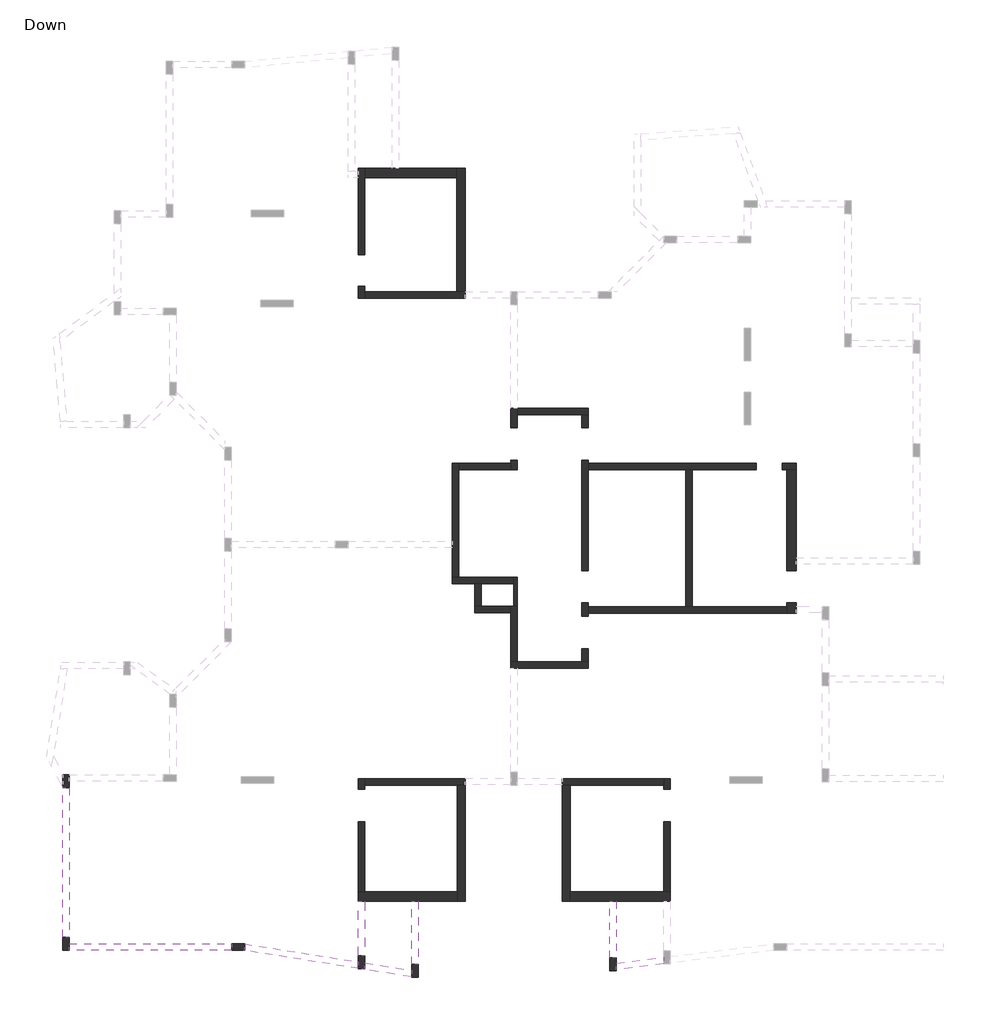
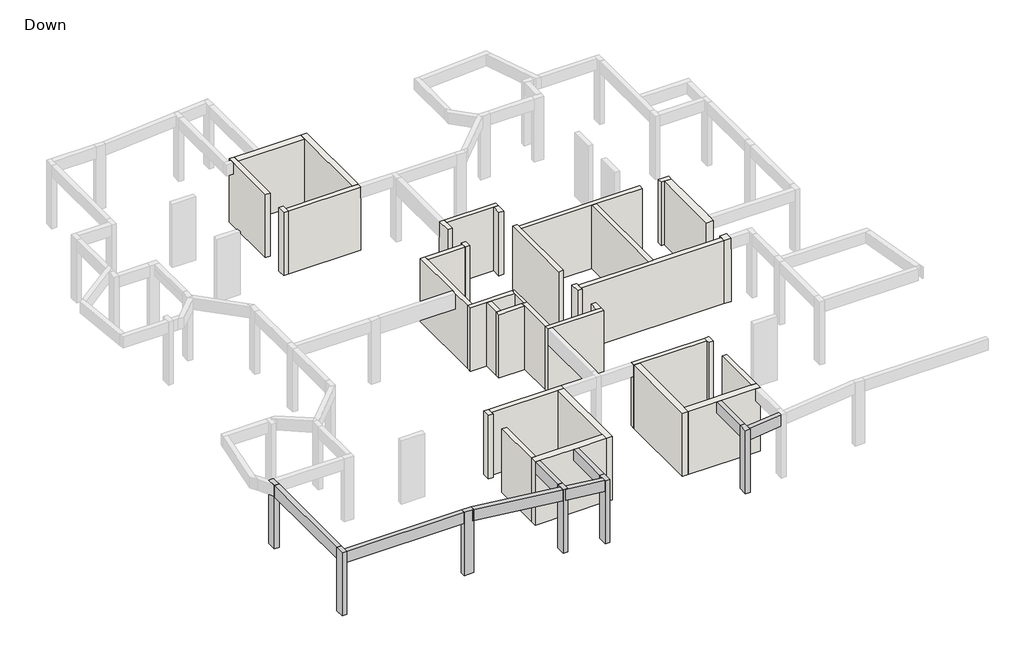
# One storey, part 1 of 3: 36 walls, 8 beams, 6 columns.
# Revit data of these elements (continued)
# Element 33 (IfcWall, "20") (continued)
#   Materials on its faces: "Concrete"
# Element 34 (IfcWall, "20")
#   Comments = ""
#   Mark = "W19"
#   SOFiSTiK_EdgeZones = "W20"
#   SOFiSTiK_AMG_Comments = ""
#   Top Offset = 0 cm
#   Base Offset = 0 cm
#   wall height = 285 cm
#   SOFiSTiK_AMG_Scheduled = yes
#   SOFiSTiK_AMG_Adjusted = yes
#   Phase Created = New Construction
#   Base Constraint = Down
#   Top Constraint = Typical Floor
#   Materials on its faces: "Concrete"
# Element 35 (IfcWall, "20")
#   Comments = ""
#   Mark = "W20"
#   SOFiSTiK_EdgeZones = "W21"
#   SOFiSTiK_AMG_Comments = ""
#   Top Offset = 0 cm
#   Base Offset = 0 cm
#   wall height = 285 cm
#   SOFiSTiK_AMG_Scheduled = yes
#   SOFiSTiK_AMG_Adjusted = yes
#   Phase Created = New Construction
#   Base Constraint = Down
#   Top Constraint = Typical Floor
#   Materials on its faces: "Concrete"
# Element 36 (IfcWall, "20")
#   Comments = ""
#   Mark = "W21"
#   SOFiSTiK_EdgeZones = "W22"
#   SOFiSTiK_AMG_Comments = ""
#   Top Offset = 0 cm
#   Base Offset = 0 cm
#   wall height = 285 cm
#   SOFiSTiK_AMG_Scheduled = yes
#   SOFiSTiK_AMG_Adjusted = yes
#   Phase Created = New Construction
#   Base Constraint = Down
#   Top Constraint = Typical Floor
#   Materials on its faces: "Concrete"
# Element 37 (IfcWall, "20")
#   Comments = ""
#   Mark = "W22"
#   SOFiSTiK_EdgeZones = "W23"
#   SOFiSTiK_AMG_Comments = ""
#   Top Offset = 0 cm
#   Base Offset = 0 cm
#   wall height = 285 cm
#   SOFiSTiK_AMG_Scheduled = yes
#   SOFiSTiK_AMG_Adjusted = yes
#   Phase Created = New Construction
#   Base Constraint = Down
#   Top Constraint = Typical Floor
#   Materials on its faces: "Concrete"
# Element 38 (IfcWall, "20")
#   Comments = ""
#   Mark = "W23"
#   SOFiSTiK_EdgeZones = "W24"
#   SOFiSTiK_AMG_Comments = ""
#   Top Offset = 0 cm
#   Base Offset = 0 cm
#   wall height = 285 cm
#   SOFiSTiK_AMG_Scheduled = yes
#   SOFiSTiK_AMG_Adjusted = yes
#   Phase Created = New Construction
#   Base Constraint = Down
#   Top Constraint = Typical Floor
#   Materials on its faces: "Concrete"
# Element 39 (IfcWall, "20")
#   Comments = ""
#   Mark = "W24"
#   SOFiSTiK_EdgeZones = "W25"
#   SOFiSTiK_AMG_Comments = ""
#   Top Offset = 0 cm
#   Base Offset = 0 cm
#   wall height = 285 cm
#   SOFiSTiK_AMG_Scheduled = yes
#   SOFiSTiK_AMG_Adjusted = yes
#   Phase Created = New Construction
#   Base Constraint = Down
#   Top Constraint = Typical Floor
#   Materials on its faces: "Concrete"
# Element 40 (IfcWall, "20")
#   Comments = ""
#   Mark = "W25"
#   SOFiSTiK_EdgeZones = "W26"
#   SOFiSTiK_AMG_Comments = ""
#   Top Offset = 0 cm
#   Base Offset = 0 cm
#   wall height = 285 cm
#   SOFiSTiK_AMG_Scheduled = yes
#   SOFiSTiK_AMG_Adjusted = yes
#   Phase Created = New Construction
#   Base Constraint = Down
#   Top Constraint = Typical Floor
#   Materials on its faces: "Concrete"
# Element 41 (IfcWall, "20")
#   Comments = ""
#   Mark = "W26"
#   SOFiSTiK_EdgeZones = "W27"
#   SOFiSTiK_AMG_Comments = ""
#   Top Offset = 0 cm
#   Base Offset = 0 cm
#   wall height = 285 cm
#   SOFiSTiK_AMG_Scheduled = yes
#   SOFiSTiK_AMG_Adjusted = yes
#   Phase Created = New Construction
#   Base Constraint = Down
#   Top Constraint = Typical Floor
#   Materials on its faces: "Concrete"
# Element 42 (IfcWall, "20")
#   Comments = ""
#   Mark = "W27"
#   SOFiSTiK_EdgeZones = "W28"
#   SOFiSTiK_AMG_Comments = ""
#   Top Offset = 0 cm
#   Base Offset = 0 cm
#   wall height = 285 cm
#   SOFiSTiK_AMG_Scheduled = yes
#   SOFiSTiK_AMG_Adjusted = yes
#   Phase Created = New Construction
#   Base Constraint = Down
#   Top Constraint = Typical Floor
#   Materials on its faces: "Concrete"
# Element 43 (IfcWall, "25")
#   Comments = ""
#   Mark = "W28"
#   SOFiSTiK_EdgeZones = "W29"
#   SOFiSTiK_AMG_Comments = ""
#   Top Offset = 0 cm
#   Base Offset = 0 cm
#   wall height = 285 cm
#   SOFiSTiK_AMG_Scheduled = yes
#   SOFiSTiK_AMG_Adjusted = yes
#   Phase Created = New Construction
#   Base Constraint = Down
#   Top Constraint = Typical Floor
#   Materials on its faces: "Concrete"
# Element 44 (IfcWall, "25")
#   Comments = ""
#   Mark = "W29"
#   SOFiSTiK_EdgeZones = "W30"
#   SOFiSTiK_AMG_Comments = ""
#   Top Offset = 0 cm
#   Base Offset = 0 cm
#   wall height = 285 cm
#   SOFiSTiK_AMG_Scheduled = yes
#   SOFiSTiK_AMG_Adjusted = yes
#   Phase Created = New Construction
#   Base Constraint = Down
#   Top Constraint = Typical Floor
#   Materials on its faces: "Concrete"
# Element 45 (IfcWall, "25")
#   Comments = ""
#   Mark = "W30"
#   SOFiSTiK_EdgeZones = "W31"
#   SOFiSTiK_AMG_Comments = ""
#   Top Offset = 0 cm
#   Base Offset = 0 cm
#   wall height = 285 cm
#   SOFiSTiK_AMG_Scheduled = yes
#   SOFiSTiK_AMG_Adjusted = yes
#   Phase Created = New Construction
#   Base Constraint = Down
#   Top Constraint = Typical Floor
#   Materials on its faces: "Concrete"
# Element 46 (IfcWall, "30")
#   Comments = ""
#   Mark = "W31"
#   SOFiSTiK_EdgeZones = "W32"
#   SOFiSTiK_AMG_Comments = ""
#   Top Offset = 0 cm
#   Base Offset = 0 cm
#   wall height = 285 cm
#   SOFiSTiK_AMG_Scheduled = yes
#   SOFiSTiK_AMG_Adjusted = yes
#   Phase Created = New Construction
#   Base Constraint = Down
#   Top Constraint = Typical Floor
#   Materials on its faces: "Concrete"
# Element 47 (IfcWall, "30")
#   Comments = ""
#   Mark = "W32"
#   SOFiSTiK_EdgeZones = "W33"
#   SOFiSTiK_AMG_Comments = ""
#   Top Offset = 0 cm
#   Base Offset = 0 cm
#   wall height = 285 cm
#   SOFiSTiK_AMG_Scheduled = yes
#   SOFiSTiK_AMG_Adjusted = yes
#   Phase Created = New Construction
#   Base Constraint = Down
#   Top Constraint = Typical Floor
#   Materials on its faces: "Concrete"
# Element 48 (IfcWall, "30")
#   Comments = ""
#   Mark = "W33"
#   SOFiSTiK_EdgeZones = "W34"
#   SOFiSTiK_AMG_Comments = ""
#   Top Offset = 0 cm
#   Base Offset = 0 cm
#   wall height = 285 cm
#   SOFiSTiK_AMG_Scheduled = yes
#   SOFiSTiK_AMG_Adjusted = yes
#   Phase Created = New Construction
#   Base Constraint = Down
#   Top Constraint = Typical Floor
#   Materials on its faces: "Concrete"
# Element 49 (IfcWall, "30")
#   Comments = ""
#   Mark = "W34"
#   SOFiSTiK_EdgeZones = "W35"
#   SOFiSTiK_AMG_Comments = ""
#   Top Offset = 0 cm
#   Base Offset = 0 cm
#   wall height = 285 cm
#   SOFiSTiK_AMG_Scheduled = yes
#   SOFiSTiK_AMG_Adjusted = yes
#   Phase Created = New Construction
#   Base Constraint = Down
#   Top Constraint = Typical Floor
#   Materials on its faces: "Concrete"
# Element 50 (IfcWall, "30")
#   Comments = ""
#   Mark = "W35"
#   SOFiSTiK_EdgeZones = "W36"
#   SOFiSTiK_AMG_Comments = ""
#   Top Offset = 0 cm
#   Base Offset = 0 cm
#   wall height = 285 cm
#   SOFiSTiK_AMG_Scheduled = yes
#   SOFiSTiK_AMG_Adjusted = yes
#   Phase Created = New Construction
#   Base Constraint = Down
#   Top Constraint = Typical Floor
#   Materials on its faces: "Concrete"
# Materials
#   "Concrete": class "Concrete", colour RGB 192 192 192, transparency 0, Keynote = "01000", Description = "Cast-in-place concrete", Cost = 0
